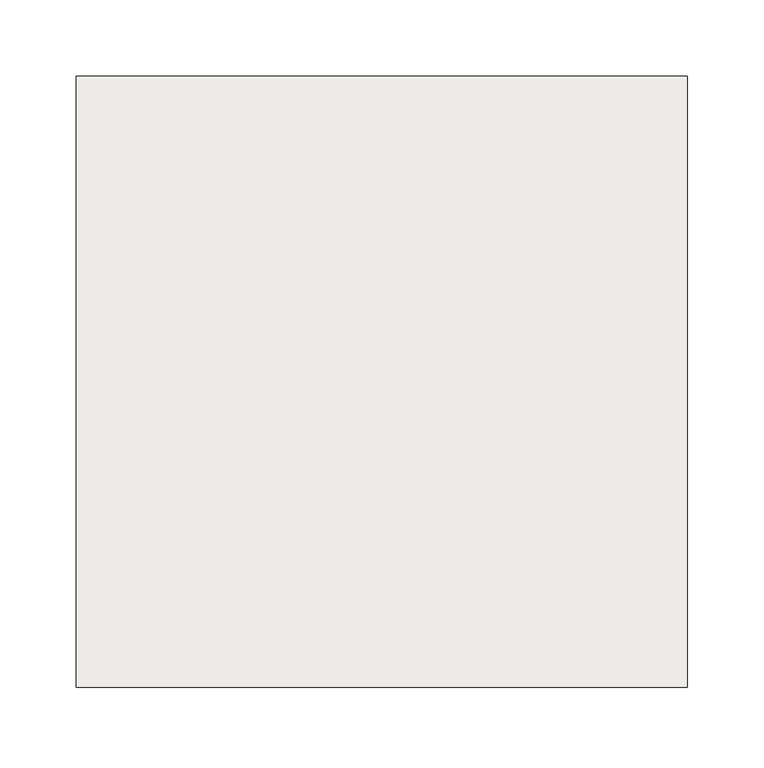
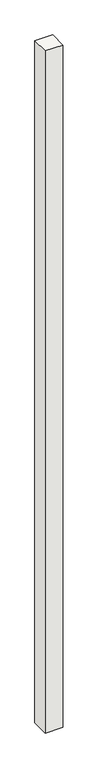
"""IFC4 building model written with IfcOpenShell, lengths in millimetres: slab geometry, NLRS_17_SFO_TLB_funderingspaal geheid beton prefab-AV-MMBPC_gen_rsf : heipaal beton prefab_gen__bxh 400x400."""

from ifc_helpers import new_model, si_unit, frame, origin, place, context, project, spatial, polyline, outline, extrude, source, transform, mapped, element, save


def slab_d279473c(model_context):
    return source(origin(), model_context, "Body", "SweptSolid", [
        extrude(outline(polyline([(200.0, -200.0), (-200.0, -200.0), (-200.0, 200.0), (200.0, 200.0), (200.0, -200.0)])), frame((0.0, 0.0, -20000.0), z_axis=(0.0, 0.0, 1.0), x_axis=(1.0, 0.0, 0.0)), (0.0, 0.0, 1.0), 16250.0),
    ])


if __name__ == "__main__":
    model = new_model("IFC4")
    model_context = context("Model", 3, world=origin())
    ifc_project = project(units=[si_unit("LENGTHUNIT", "METRE", prefix="MILLI")], contexts=[model_context])
    site = spatial("IfcSite", under=ifc_project)
    building = spatial("IfcBuilding", under=site)
    placement = place(None, origin())
    slab_shape = slab_d279473c(model_context)
    element("IfcSlab", 1, ObjectType="NLRS_17_SFO_TLB_funderingspaal geheid beton prefab-AV-MMBPC_gen_rsf : heipaal beton prefab_gen__bxh 400x400", at=placement, inside=building, context=model_context, shape_type="MappedRepresentation", body=[
        mapped(slab_shape, transform((0.0, 0.0, 0.0), x_axis=(1.0, 0.0, 0.0), y_axis=(0.0, 1.0, 0.0), z_axis=(0.0, 0.0, 1.0))),
    ])
    save(model, "model.ifc")

# Revit data of these elements
# Type "NLRS_17_SFO_TLB_funderingspaal geheid beton prefab-AV-MMBPC_gen_rsf : heipaal beton prefab_gen__bxh 400x400"
#   Export Type to IFC As = "IfcPile"
#   Type IfcGUID = "10$Kfo5uPCAOPJEOo5LE_W"
#   Type Comments = "prefab heipaal 400x400"
#   Model = " "
#   Manufacturer = " "
#   Description = "prefab heipaal 400x400"
#   Assembly Code = "17.21"
#   Width = 400 mm
#   Slanted Angle [instance default] = 0.00°
#   NLRS_S_draagvermogen_trek [instance default] = 0.00 kN
#   NLRS_S_draagvermogen_druk [instance default] = 0.00 kN
#   NLRS_C_lengte [instance default] = 1660 mm
#   NLRS_C_hoogte = 400 mm
#   NLRS_C_breedte = 400 mm
#   Height [instance default] = 1660 mm
#   Length [instance default] = 1660 mm
#   Angle [instance default] = 0.00°
#   Slanted [instance default] = 0
#   Structural Material = NLRS_f2_beton prefab_gen_rsf
#   Keynote = ""
# Element 1 (IfcSlab, "NLRS_17_SFO_TLB_funderingspaal geheid beton prefab-AV-MMBPC_gen_rsf : heipaal beton prefab_gen__bxh 400x400")
#   NLRS_C_lengte = 16250 mm
#   Height = 16250 mm
#   Length = 16250 mm
#   Materials on its faces: "NLRS_f2_beton prefab_gen_rsf"
# Materials
#   "NLRS_f2_beton prefab_gen_rsf": class "F - Niet gebakken kunststeen", colour RGB 129 133 118, transparency 0, Keynote = "f2", Manufacturer = "Revit Standards Foundation", URL = "www.revitstandards.org", Description = "beton prefab", Cost = 0
